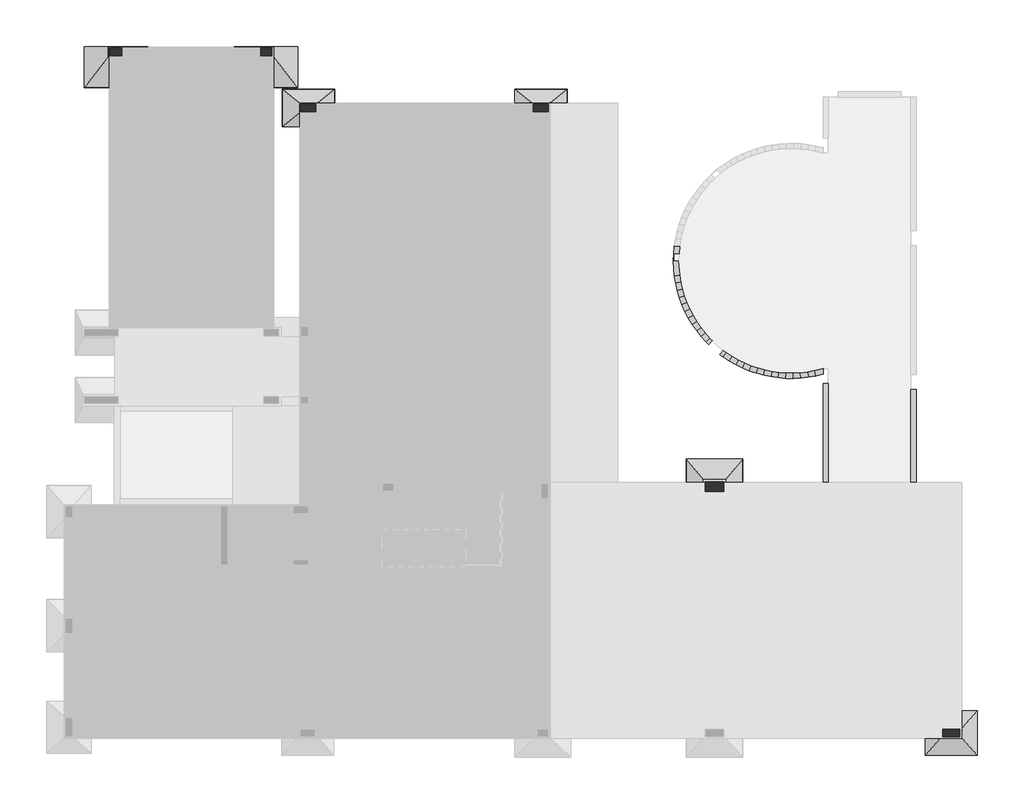
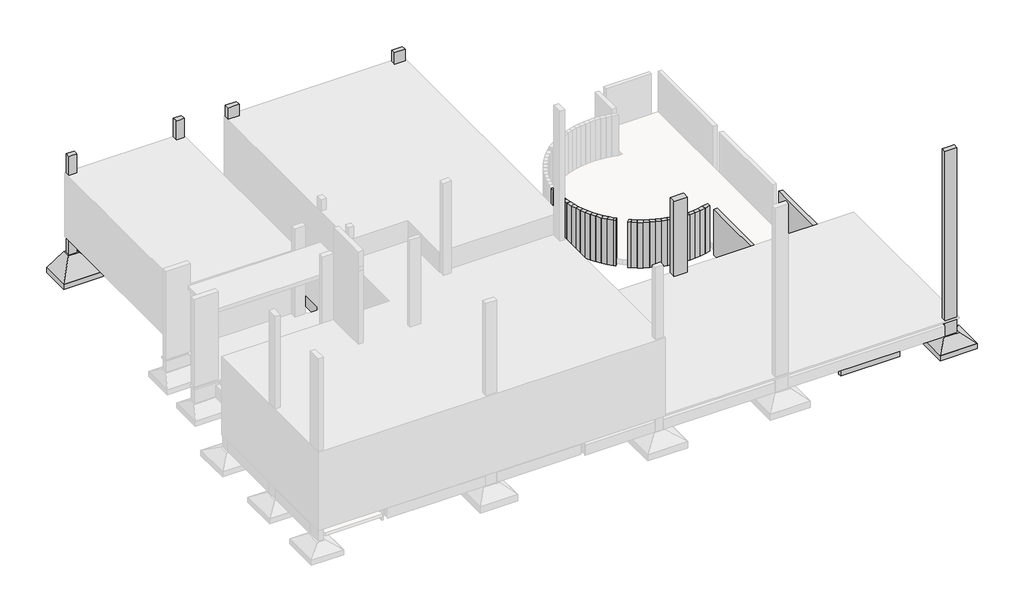
# One storey, part 3 of 4: 35 beams, 7 fasteners, 6 columns.
# Revit data of these elements (continued)
# Type "TQS - Sapata : S2" (continued)
#   H0 = 0.20 m
#   EXCYABS = 0.85 m
#   EXCY = 0.00 m
#   EXCXABS = 0.145 m
#   EXCX = -0.405 m
#   DIMY = 1.70 m
#   DIMX = 1.10 m
#   Material estrutural = Concreto - Concreto concretado no local
#   Width = 0
#   Length = 0
# Type "TQS - Sapata : S24"
#   TY = 0.60 m
#   TX = 0.29 m
#   HS = 0.50 m
#   H0 = 0.20 m
#   EXCYABS = 0.70 m
#   EXCY = 0.00 m
#   EXCXABS = 0.60 m
#   EXCX = 0.00 m
#   DIMY = 1.40 m
#   DIMX = 1.20 m
#   Material estrutural = Concreto - Concreto concretado no local
#   Width = 0
#   Length = 0
# Type "TQS - Sapata : S3"
#   TY = 0.50 m
#   TX = 0.29 m
#   HS = 0.50 m
#   H0 = 0.20 m
#   EXCYABS = 0.70 m
#   EXCY = 0.00 m
#   EXCXABS = 0.50 m
#   EXCX = 0.00 m
#   DIMY = 1.40 m
#   DIMX = 1.00 m
#   Material estrutural = Concreto - Concreto concretado no local
#   Width = 0
#   Length = 0
# Type "TQS - Sapata : S4"
#   TY = 0.50 m
#   TX = 0.29 m
#   HS = 0.50 m
#   H0 = 0.20 m
#   EXCYABS = 0.70 m
#   EXCY = 0.00 m
#   EXCXABS = 0.50 m
#   EXCX = 0.00 m
#   DIMY = 1.40 m
#   DIMX = 1.00 m
#   Material estrutural = Concreto - Concreto concretado no local
#   Width = 0
#   Length = 0
# Element 1 (IfcBeam, "TQS - Viga retangular : 14.0 x 180.0")
#   Uso = "ESTRUTURA"
#   Titulo = "VP2"
#   Chave = "-984"
#   Tipo Elemento = "Viga"
#   SHA1 = "67BB47F7F07D141E1E461B1B62FFCED57BE49A5E"
#   Revisão = ""
#   Tipo de carga = ""
#   Divisor de flexao = ""
#   Secao = ""
#   Configuracao = ""
#   Angulo (graus) = ""
#   Detalhamento = ""
#   Casos de vento manual = ""
#   Tipo = ""
#   Alcas = ""
#   Furos = ""
#   Pino = ""
#   Distribuicao = ""
#   Solidarizado = ""
#   Solidarizar na montagem = ""
#   Unir com o próximo = ""
#   Grupo pre moldado = ""
#   Verificado = ""
#   Concreto C = ""
#   Taxa de armadura (kgf/m³) = 0
#   Carga (tf/m²) = 0
#   Carga (tf/m) = 0
#   Carga (tf) = 0
#   Altura = 1.80 m
#   Rebaixo = 0.15 m
#   Largura = 0.14 m
#   Distancia a face = 0.00 m
#   Distancia ao eixo = 0.00 m
#   Altura gerber esquerda = 0.00 m
#   Largura gerber esquerda = 0.00 m
#   Altura gerber direita = 0.00 m
#   Largura gerber direita = 0.00 m
#   Resultado de Ensaios fck (MPa) = 0
#   Unique TQS ID = -984
#   Principal = yes
#   Structural Material = none
#   Phase Created = CC_AP/ESTR
# Element 2 (IfcBeam, "TQS - Viga retangular : 14.0 x 180.0")
#   Uso = "ESTRUTURA"
#   Titulo = "VP3"
#   Chave = "-985"
#   Tipo Elemento = "Viga"
#   SHA1 = "1D3F2A738C11C779DD3B877E14C8E10A324E012C"
#   Revisão = ""
#   Tipo de carga = ""
#   Divisor de flexao = ""
#   Secao = ""
#   Configuracao = ""
#   Angulo (graus) = ""
#   Detalhamento = ""
#   Casos de vento manual = ""
#   Tipo = ""
#   Alcas = ""
#   Furos = ""
#   Pino = ""
#   Distribuicao = ""
#   Solidarizado = ""
#   Solidarizar na montagem = ""
#   Unir com o próximo = ""
#   Grupo pre moldado = ""
#   Verificado = ""
#   Concreto C = ""
#   Taxa de armadura (kgf/m³) = 0
#   Carga (tf/m²) = 0
#   Carga (tf/m) = 0
#   Carga (tf) = 0
#   Altura = 1.80 m
#   Rebaixo = 0.15 m
#   Largura = 0.14 m
#   Distancia a face = 0.00 m
#   Distancia ao eixo = 0.00 m
#   Altura gerber esquerda = 0.00 m
#   Largura gerber esquerda = 0.00 m
#   Altura gerber direita = 0.00 m
#   Largura gerber direita = 0.00 m
#   Resultado de Ensaios fck (MPa) = 0
#   Unique TQS ID = -985
#   Principal = yes
#   Structural Material = none
#   Phase Created = CC_AP/ESTR
# Element 3 (IfcBeam, "TQS - Viga retangular : 14.0 x 180.0")
#   Uso = "ESTRUTURA"
#   Titulo = "VP4"
#   Chave = "-987"
#   Tipo Elemento = "Viga"
#   SHA1 = "18E803970E3FF61AE3A7C4B8095E8E40226C0AA9"
#   Revisão = ""
#   Tipo de carga = ""
#   Divisor de flexao = ""
#   Secao = ""
#   Configuracao = ""
#   Angulo (graus) = ""
#   Detalhamento = ""
#   Casos de vento manual = ""
#   Tipo = ""
#   Alcas = ""
#   Furos = ""
#   Pino = ""
#   Distribuicao = ""
#   Solidarizado = ""
#   Solidarizar na montagem = ""
#   Unir com o próximo = ""
#   Grupo pre moldado = ""
#   Verificado = ""
#   Concreto C = ""
#   Taxa de armadura (kgf/m³) = 0
#   Carga (tf/m²) = 0
#   Carga (tf/m) = 0
#   Carga (tf) = 0
#   Altura = 1.80 m
#   Rebaixo = 0.15 m
#   Largura = 0.14 m
#   Distancia a face = 0.00 m
#   Distancia ao eixo = 0.00 m
#   Altura gerber esquerda = 0.00 m
#   Largura gerber esquerda = 0.00 m
#   Altura gerber direita = 0.00 m
#   Largura gerber direita = 0.00 m
#   Resultado de Ensaios fck (MPa) = 0
#   Unique TQS ID = -987
#   Principal = yes
#   Structural Material = none
#   Phase Created = CC_AP/ESTR
# Element 4 (IfcBeam, "TQS - Viga retangular : 14.0 x 180.0")
#   Uso = "ESTRUTURA"
#   Titulo = "VP4"
#   Chave = "-988"
#   Tipo Elemento = "Viga"
#   SHA1 = "B71FF30D7224BC3A2F9C0912C04A339394FFFF18"
#   Revisão = ""
#   Tipo de carga = ""
#   Divisor de flexao = ""
#   Secao = ""
#   Configuracao = ""
#   Angulo (graus) = ""
#   Detalhamento = ""
#   Casos de vento manual = ""
#   Tipo = ""
#   Alcas = ""
#   Furos = ""
#   Pino = ""
#   Distribuicao = ""
#   Solidarizado = ""
#   Solidarizar na montagem = ""
#   Unir com o próximo = ""
#   Grupo pre moldado = ""
#   Verificado = ""
#   Concreto C = ""
#   Taxa de armadura (kgf/m³) = 0
#   Carga (tf/m²) = 0
#   Carga (tf/m) = 0
#   Carga (tf) = 0
#   Altura = 1.80 m
#   Rebaixo = 0.15 m
#   Largura = 0.14 m
#   Distancia a face = 0.00 m
#   Distancia ao eixo = 0.00 m
#   Altura gerber esquerda = 0.00 m
#   Largura gerber esquerda = 0.00 m
#   Altura gerber direita = 0.00 m
#   Largura gerber direita = 0.00 m
#   Resultado de Ensaios fck (MPa) = 0
#   Unique TQS ID = -988
#   Principal = yes
#   Structural Material = none
#   Phase Created = CC_AP/ESTR
# Element 5 (IfcBeam, "TQS - Viga retangular : 14.0 x 180.0")
#   Uso = "ESTRUTURA"
#   Titulo = "VP4"
#   Chave = "-989"
#   Tipo Elemento = "Viga"
#   SHA1 = "E9E1B2FEFAB6FC9E808C50FA3A91823AD53CDAD9"
#   Revisão = ""
#   Tipo de carga = ""
#   Divisor de flexao = ""
#   Secao = ""
#   Configuracao = ""
#   Angulo (graus) = ""
#   Detalhamento = ""
#   Casos de vento manual = ""
#   Tipo = ""
#   Alcas = ""
#   Furos = ""
#   Pino = ""
#   Distribuicao = ""
#   Solidarizado = ""
#   Solidarizar na montagem = ""
#   Unir com o próximo = ""
#   Grupo pre moldado = ""
#   Verificado = ""
#   Concreto C = ""
#   Taxa de armadura (kgf/m³) = 0
#   Carga (tf/m²) = 0
#   Carga (tf/m) = 0
#   Carga (tf) = 0
#   Altura = 1.80 m
#   Rebaixo = 0.15 m
#   Largura = 0.14 m
#   Distancia a face = 0.00 m
#   Distancia ao eixo = 0.00 m
#   Altura gerber esquerda = 0.00 m
#   Largura gerber esquerda = 0.00 m
#   Altura gerber direita = 0.00 m
#   Largura gerber direita = 0.00 m
#   Resultado de Ensaios fck (MPa) = 0
#   Unique TQS ID = -989
#   Principal = yes
#   Structural Material = none
#   Phase Created = CC_AP/ESTR
# Element 6 (IfcBeam, "TQS - Viga retangular : 14.0 x 180.0")
#   Uso = "ESTRUTURA"
#   Titulo = "VP4"
#   Chave = "-990"
#   Tipo Elemento = "Viga"
#   SHA1 = "A4F79934EF83F3B7E9A1E2CD35D009C4681F812D"
#   Revisão = ""
#   Tipo de carga = ""
#   Divisor de flexao = ""
#   Secao = ""
#   Configuracao = ""
#   Angulo (graus) = ""
#   Detalhamento = ""
#   Casos de vento manual = ""
#   Tipo = ""
#   Alcas = ""
#   Furos = ""
#   Pino = ""
#   Distribuicao = ""
#   Solidarizado = ""
#   Solidarizar na montagem = ""
#   Unir com o próximo = ""
#   Grupo pre moldado = ""
#   Verificado = ""
#   Concreto C = ""
#   Taxa de armadura (kgf/m³) = 0
#   Carga (tf/m²) = 0
#   Carga (tf/m) = 0
#   Carga (tf) = 0
#   Altura = 1.80 m
#   Rebaixo = 0.15 m
#   Largura = 0.14 m
#   Distancia a face = 0.00 m
#   Distancia ao eixo = 0.00 m
#   Altura gerber esquerda = 0.00 m
#   Largura gerber esquerda = 0.00 m
#   Altura gerber direita = 0.00 m
#   Largura gerber direita = 0.00 m
#   Resultado de Ensaios fck (MPa) = 0
#   Unique TQS ID = -990
#   Principal = yes
#   Structural Material = none
#   Phase Created = CC_AP/ESTR
# Element 7 (IfcBeam, "TQS - Viga retangular : 14.0 x 180.0")
#   Uso = "ESTRUTURA"
#   Titulo = "VP4"
#   Chave = "-991"
#   Tipo Elemento = "Viga"
#   SHA1 = "59C2882C15F8D77C9BC823B17A9B229971BFE292"
#   Revisão = ""
#   Tipo de carga = ""
#   Divisor de flexao = ""
#   Secao = ""
#   Configuracao = ""
#   Angulo (graus) = ""
#   Detalhamento = ""
#   Casos de vento manual = ""
#   Tipo = ""
#   Alcas = ""
#   Furos = ""
#   Pino = ""
#   Distribuicao = ""
#   Solidarizado = ""
#   Solidarizar na montagem = ""
#   Unir com o próximo = ""
#   Grupo pre moldado = ""
#   Verificado = ""
#   Concreto C = ""
#   Taxa de armadura (kgf/m³) = 0
#   Carga (tf/m²) = 0
#   Carga (tf/m) = 0
#   Carga (tf) = 0
#   Altura = 1.80 m
#   Rebaixo = 0.15 m
#   Largura = 0.14 m
#   Distancia a face = 0.00 m
#   Distancia ao eixo = 0.00 m
#   Altura gerber esquerda = 0.00 m
#   Largura gerber esquerda = 0.00 m
#   Altura gerber direita = 0.00 m
#   Largura gerber direita = 0.00 m
#   Resultado de Ensaios fck (MPa) = 0
#   Unique TQS ID = -991
#   Principal = yes
#   Structural Material = none
#   Phase Created = CC_AP/ESTR
# Element 8 (IfcBeam, "TQS - Viga retangular : 14.0 x 180.0")
#   Uso = "ESTRUTURA"
#   Titulo = "VP4"
#   Chave = "-992"
#   Tipo Elemento = "Viga"
#   SHA1 = "6D985E6B9F5FA1FD140F505980BE925AA5C487F2"
#   Revisão = ""
#   Tipo de carga = ""
#   Divisor de flexao = ""
#   Secao = ""
#   Configuracao = ""
#   Angulo (graus) = ""
#   Detalhamento = ""
#   Casos de vento manual = ""
#   Tipo = ""
#   Alcas = ""
#   Furos = ""
#   Pino = ""
#   Distribuicao = ""
#   Solidarizado = ""
#   Solidarizar na montagem = ""
#   Unir com o próximo = ""
#   Grupo pre moldado = ""
#   Verificado = ""
#   Concreto C = ""
#   Taxa de armadura (kgf/m³) = 0
#   Carga (tf/m²) = 0
#   Carga (tf/m) = 0
#   Carga (tf) = 0
#   Altura = 1.80 m
#   Rebaixo = 0.15 m
#   Largura = 0.14 m
#   Distancia a face = 0.00 m
#   Distancia ao eixo = 0.00 m
#   Altura gerber esquerda = 0.00 m
#   Largura gerber esquerda = 0.00 m
#   Altura gerber direita = 0.00 m
#   Largura gerber direita = 0.00 m
#   Resultado de Ensaios fck (MPa) = 0
#   Unique TQS ID = -992
#   Principal = yes
#   Structural Material = none
#   Phase Created = CC_AP/ESTR
# Element 9 (IfcBeam, "TQS - Viga retangular : 14.0 x 180.0")
#   Uso = "ESTRUTURA"
#   Titulo = "VP4"
#   Chave = "-993"
#   Tipo Elemento = "Viga"
#   SHA1 = "5D4E92287FB362FDFCD64B2B7E6C35302CB92A79"
#   Revisão = ""
#   Tipo de carga = ""
#   Divisor de flexao = ""
#   Secao = ""
#   Configuracao = ""
#   Angulo (graus) = ""
#   Detalhamento = ""
#   Casos de vento manual = ""
#   Tipo = ""
#   Alcas = ""
#   Furos = ""
#   Pino = ""
#   Distribuicao = ""
#   Solidarizado = ""
#   Solidarizar na montagem = ""
#   Unir com o próximo = ""
#   Grupo pre moldado = ""
#   Verificado = ""
#   Concreto C = ""
#   Taxa de armadura (kgf/m³) = 0
#   Carga (tf/m²) = 0
#   Carga (tf/m) = 0
#   Carga (tf) = 0
#   Altura = 1.80 m
#   Rebaixo = 0.15 m
#   Largura = 0.14 m
#   Distancia a face = 0.00 m
#   Distancia ao eixo = 0.00 m
#   Altura gerber esquerda = 0.00 m
#   Largura gerber esquerda = 0.00 m
#   Altura gerber direita = 0.00 m
#   Largura gerber direita = 0.00 m
#   Resultado de Ensaios fck (MPa) = 0
#   Unique TQS ID = -993
#   Principal = yes
#   Structural Material = none
#   Phase Created = CC_AP/ESTR
# Element 10 (IfcBeam, "TQS - Viga retangular : 14.0 x 180.0")
#   Uso = "ESTRUTURA"
#   Titulo = "VP4"
#   Chave = "-994"
#   Tipo Elemento = "Viga"
#   SHA1 = "B241F61C6536B176DF9E3A8727FE075D16BE7057"
#   Revisão = ""
#   Tipo de carga = ""
#   Divisor de flexao = ""
#   Secao = ""
#   Configuracao = ""
#   Angulo (graus) = ""
#   Detalhamento = ""
#   Casos de vento manual = ""
#   Tipo = ""
#   Alcas = ""
#   Furos = ""
#   Pino = ""
#   Distribuicao = ""
#   Solidarizado = ""
#   Solidarizar na montagem = ""
#   Unir com o próximo = ""
#   Grupo pre moldado = ""
#   Verificado = ""
#   Concreto C = ""
#   Taxa de armadura (kgf/m³) = 0
#   Carga (tf/m²) = 0
#   Carga (tf/m) = 0
#   Carga (tf) = 0
#   Altura = 1.80 m
#   Rebaixo = 0.15 m
#   Largura = 0.14 m
#   Distancia a face = 0.00 m
#   Distancia ao eixo = 0.00 m
#   Altura gerber esquerda = 0.00 m
#   Largura gerber esquerda = 0.00 m
#   Altura gerber direita = 0.00 m
#   Largura gerber direita = 0.00 m
#   Resultado de Ensaios fck (MPa) = 0
#   Unique TQS ID = -994
#   Principal = yes
#   Structural Material = none
#   Phase Created = CC_AP/ESTR
# Element 11 (IfcBeam, "TQS - Viga retangular : 14.0 x 180.0")
#   Uso = "ESTRUTURA"
#   Titulo = "VP4"
#   Chave = "-995"
#   Tipo Elemento = "Viga"
#   SHA1 = "79F2E8F443EC2E8CC5B8F506A3E5025E7F953CE7"
#   Revisão = ""
#   Tipo de carga = ""
#   Divisor de flexao = ""
#   Secao = ""
#   Configuracao = ""
#   Angulo (graus) = ""
#   Detalhamento = ""
#   Casos de vento manual = ""
#   Tipo = ""
#   Alcas = ""
#   Furos = ""
#   Pino = ""
#   Distribuicao = ""
#   Solidarizado = ""
#   Solidarizar na montagem = ""
#   Unir com o próximo = ""
#   Grupo pre moldado = ""
#   Verificado = ""
#   Concreto C = ""
#   Taxa de armadura (kgf/m³) = 0
#   Carga (tf/m²) = 0
#   Carga (tf/m) = 0
#   Carga (tf) = 0
#   Altura = 1.80 m
#   Rebaixo = 0.15 m
#   Largura = 0.14 m
#   Distancia a face = 0.00 m
#   Distancia ao eixo = 0.00 m
#   Altura gerber esquerda = 0.00 m
#   Largura gerber esquerda = 0.00 m
#   Altura gerber direita = 0.00 m
#   Largura gerber direita = 0.00 m
#   Resultado de Ensaios fck (MPa) = 0
#   Unique TQS ID = -995
#   Principal = yes
#   Structural Material = none
#   Phase Created = CC_AP/ESTR
# Element 12 (IfcBeam, "TQS - Viga retangular : 14.0 x 180.0")
#   Uso = "ESTRUTURA"
#   Titulo = "VP4"
#   Chave = "-996"
#   Tipo Elemento = "Viga"
#   SHA1 = "EC69CF733B6B75DD72A616518C986B1D4EC6373A"
#   Revisão = ""
#   Tipo de carga = ""
#   Divisor de flexao = ""
#   Secao = ""
#   Configuracao = ""
#   Angulo (graus) = ""
#   Detalhamento = ""
#   Casos de vento manual = ""
#   Tipo = ""
#   Alcas = ""
#   Furos = ""
#   Pino = ""
#   Distribuicao = ""
#   Solidarizado = ""
#   Solidarizar na montagem = ""
#   Unir com o próximo = ""
#   Grupo pre moldado = ""
#   Verificado = ""
#   Concreto C = ""
#   Taxa de armadura (kgf/m³) = 0
#   Carga (tf/m²) = 0
#   Carga (tf/m) = 0
#   Carga (tf) = 0
#   Altura = 1.80 m
#   Rebaixo = 0.15 m
#   Largura = 0.14 m
#   Distancia a face = 0.00 m
#   Distancia ao eixo = 0.00 m
#   Altura gerber esquerda = 0.00 m
#   Largura gerber esquerda = 0.00 m
#   Altura gerber direita = 0.00 m
#   Largura gerber direita = 0.00 m
#   Resultado de Ensaios fck (MPa) = 0
#   Unique TQS ID = -996
#   Principal = yes
#   Structural Material = none
#   Phase Created = CC_AP/ESTR
# Element 13 (IfcBeam, "TQS - Viga retangular : 14.0 x 180.0")
#   Uso = "ESTRUTURA"
#   Titulo = "VP4"
#   Chave = "-997"
#   Tipo Elemento = "Viga"
#   SHA1 = "A94BB0AB94C95055560F49AF3BCE408F9E38B8C0"
#   Revisão = ""
#   Tipo de carga = ""
#   Divisor de flexao = ""
#   Secao = ""
#   Configuracao = ""
#   Angulo (graus) = ""
#   Detalhamento = ""
#   Casos de vento manual = ""
#   Tipo = ""
#   Alcas = ""
#   Furos = ""
#   Pino = ""
#   Distribuicao = ""
#   Solidarizado = ""
#   Solidarizar na montagem = ""
#   Unir com o próximo = ""
#   Grupo pre moldado = ""
#   Verificado = ""
#   Concreto C = ""
#   Taxa de armadura (kgf/m³) = 0
#   Carga (tf/m²) = 0
#   Carga (tf/m) = 0
#   Carga (tf) = 0
#   Altura = 1.80 m
#   Rebaixo = 0.15 m
#   Largura = 0.14 m
#   Distancia a face = 0.00 m
#   Distancia ao eixo = 0.00 m
#   Altura gerber esquerda = 0.00 m
#   Largura gerber esquerda = 0.00 m
#   Altura gerber direita = 0.00 m
#   Largura gerber direita = 0.00 m
#   Resultado de Ensaios fck (MPa) = 0
#   Unique TQS ID = -997
#   Principal = yes
#   Structural Material = none
#   Phase Created = CC_AP/ESTR
# Element 14 (IfcBeam, "TQS - Viga retangular : 14.0 x 180.0")
#   Uso = "ESTRUTURA"
#   Titulo = "VP4"
#   Chave = "-998"
#   Tipo Elemento = "Viga"
#   SHA1 = "6378FB8D39603434150BF0AD569D703CFB80FE5F"
#   Revisão = ""
#   Tipo de carga = ""
#   Divisor de flexao = ""
#   Secao = ""
#   Configuracao = ""
#   Angulo (graus) = ""
#   Detalhamento = ""
#   Casos de vento manual = ""
#   Tipo = ""
#   Alcas = ""
#   Furos = ""
#   Pino = ""
#   Distribuicao = ""
#   Solidarizado = ""
#   Solidarizar na montagem = ""
#   Unir com o próximo = ""
#   Grupo pre moldado = ""
#   Verificado = ""
#   Concreto C = ""
#   Taxa de armadura (kgf/m³) = 0
#   Carga (tf/m²) = 0
#   Carga (tf/m) = 0
#   Carga (tf) = 0
#   Altura = 1.80 m
#   Rebaixo = 0.15 m
#   Largura = 0.14 m
#   Distancia a face = 0.00 m
#   Distancia ao eixo = 0.00 m
#   Altura gerber esquerda = 0.00 m
#   Largura gerber esquerda = 0.00 m
#   Altura gerber direita = 0.00 m
#   Largura gerber direita = 0.00 m
#   Resultado de Ensaios fck (MPa) = 0
#   Unique TQS ID = -998
#   Principal = yes
#   Structural Material = none
#   Phase Created = CC_AP/ESTR
# Element 15 (IfcBeam, "TQS - Viga retangular : 14.0 x 180.0")
#   Uso = "ESTRUTURA"
#   Titulo = "VP4"
#   Chave = "-999"
#   Tipo Elemento = "Viga"
#   SHA1 = "2B4C78D211D826E735DAAC0C825AB5B97130EBCE"
#   Revisão = ""
#   Tipo de carga = ""
#   Divisor de flexao = ""
#   Secao = ""
#   Configuracao = ""
#   Angulo (graus) = ""
#   Detalhamento = ""
#   Casos de vento manual = ""
#   Tipo = ""
#   Alcas = ""
#   Furos = ""
#   Pino = ""
#   Distribuicao = ""
#   Solidarizado = ""
#   Solidarizar na montagem = ""
#   Unir com o próximo = ""
#   Grupo pre moldado = ""
#   Verificado = ""
#   Concreto C = ""
#   Taxa de armadura (kgf/m³) = 0
#   Carga (tf/m²) = 0
#   Carga (tf/m) = 0
#   Carga (tf) = 0
#   Altura = 1.80 m
#   Rebaixo = 0.15 m
#   Largura = 0.14 m
#   Distancia a face = 0.00 m
#   Distancia ao eixo = 0.00 m
#   Altura gerber esquerda = 0.00 m
#   Largura gerber esquerda = 0.00 m
#   Altura gerber direita = 0.00 m
#   Largura gerber direita = 0.00 m
#   Resultado de Ensaios fck (MPa) = 0
#   Unique TQS ID = -999
#   Principal = yes
#   Structural Material = none
#   Phase Created = CC_AP/ESTR
# Element 16 (IfcBeam, "TQS - Viga retangular : 14.0 x 180.0")
#   Uso = "ESTRUTURA"
#   Titulo = "VP4"
#   Chave = "-1000"
#   Tipo Elemento = "Viga"
#   SHA1 = "DD50D292EAFD20D7EF85643CCD075ACF91033CA0"
#   Revisão = ""
#   Tipo de carga = ""
#   Divisor de flexao = ""
#   Secao = ""
#   Configuracao = ""
#   Angulo (graus) = ""
#   Detalhamento = ""
#   Casos de vento manual = ""
#   Tipo = ""
#   Alcas = ""
#   Furos = ""
#   Pino = ""
#   Distribuicao = ""
#   Solidarizado = ""
#   Solidarizar na montagem = ""
#   Unir com o próximo = ""
#   Grupo pre moldado = ""
#   Verificado = ""
#   Concreto C = ""
#   Taxa de armadura (kgf/m³) = 0
#   Carga (tf/m²) = 0
#   Carga (tf/m) = 0
#   Carga (tf) = 0
#   Altura = 1.80 m
#   Rebaixo = 0.15 m
#   Largura = 0.14 m
#   Distancia a face = 0.00 m
#   Distancia ao eixo = 0.00 m
#   Altura gerber esquerda = 0.00 m
#   Largura gerber esquerda = 0.00 m
#   Altura gerber direita = 0.00 m
#   Largura gerber direita = 0.00 m
#   Resultado de Ensaios fck (MPa) = 0
#   Unique TQS ID = -1000
#   Principal = yes
#   Structural Material = none
#   Phase Created = CC_AP/ESTR
# Element 17 (IfcBeam, "TQS - Viga retangular : 14.0 x 180.0")
#   Uso = "ESTRUTURA"
#   Titulo = "VP4"
#   Chave = "-1001"
#   Tipo Elemento = "Viga"
#   SHA1 = "17AE169FA700E73A155B49B14AA872A50BD18F4B"
#   Revisão = ""
#   Tipo de carga = ""
#   Divisor de flexao = ""
#   Secao = ""
#   Configuracao = ""
#   Angulo (graus) = ""
#   Detalhamento = ""
#   Casos de vento manual = ""
#   Tipo = ""
#   Alcas = ""
#   Furos = ""
#   Pino = ""
#   Distribuicao = ""
#   Solidarizado = ""
#   Solidarizar na montagem = ""
#   Unir com o próximo = ""
#   Grupo pre moldado = ""
#   Verificado = ""
#   Concreto C = ""
#   Taxa de armadura (kgf/m³) = 0
#   Carga (tf/m²) = 0
#   Carga (tf/m) = 0
#   Carga (tf) = 0
#   Altura = 1.80 m
#   Rebaixo = 0.15 m
#   Largura = 0.14 m
#   Distancia a face = 0.00 m
#   Distancia ao eixo = 0.00 m
#   Altura gerber esquerda = 0.00 m
#   Largura gerber esquerda = 0.00 m
#   Altura gerber direita = 0.00 m
#   Largura gerber direita = 0.00 m
#   Resultado de Ensaios fck (MPa) = 0
#   Unique TQS ID = -1001
#   Principal = yes
#   Structural Material = none
#   Phase Created = CC_AP/ESTR
# Element 18 (IfcBeam, "TQS - Viga retangular : 14.0 x 180.0")
#   Uso = "ESTRUTURA"
#   Titulo = "VP5"
#   Chave = "-1002"
#   Tipo Elemento = "Viga"
#   SHA1 = "4C02C5B53EDBB34F44F4EAF2E9EE20AD89CC6C79"
#   Revisão = ""
#   Tipo de carga = ""
#   Divisor de flexao = ""
#   Secao = ""
#   Configuracao = ""
#   Angulo (graus) = ""
#   Detalhamento = ""
#   Casos de vento manual = ""
#   Tipo = ""
#   Alcas = ""
#   Furos = ""
#   Pino = ""
#   Distribuicao = ""
#   Solidarizado = ""
#   Solidarizar na montagem = ""
#   Unir com o próximo = ""
#   Grupo pre moldado = ""
#   Verificado = ""
#   Concreto C = ""
#   Taxa de armadura (kgf/m³) = 0
#   Carga (tf/m²) = 0
#   Carga (tf/m) = 0
#   Carga (tf) = 0
#   Altura = 1.80 m
#   Rebaixo = 0.15 m
#   Largura = 0.14 m
#   Distancia a face = 0.00 m
#   Distancia ao eixo = 0.00 m
#   Altura gerber esquerda = 0.00 m
#   Largura gerber esquerda = 0.00 m
#   Altura gerber direita = 0.00 m
#   Largura gerber direita = 0.00 m
#   Resultado de Ensaios fck (MPa) = 0
#   Unique TQS ID = -1002
#   Principal = yes
#   Structural Material = none
#   Phase Created = CC_AP/ESTR
# Element 19 (IfcBeam, "TQS - Viga retangular : 14.0 x 180.0")
#   Uso = "ESTRUTURA"
#   Titulo = "VP5"
#   Chave = "-1003"
#   Tipo Elemento = "Viga"
#   SHA1 = "4CC80C174DC5A33A4959CFE9988141447D2CA55C"
#   Revisão = ""
#   Tipo de carga = ""
#   Divisor de flexao = ""
#   Secao = ""
#   Configuracao = ""
#   Angulo (graus) = ""
#   Detalhamento = ""
#   Casos de vento manual = ""
#   Tipo = ""
#   Alcas = ""
#   Furos = ""
#   Pino = ""
#   Distribuicao = ""
#   Solidarizado = ""
#   Solidarizar na montagem = ""
#   Unir com o próximo = ""
#   Grupo pre moldado = ""
#   Verificado = ""
#   Concreto C = ""
#   Taxa de armadura (kgf/m³) = 0
#   Carga (tf/m²) = 0
#   Carga (tf/m) = 0
#   Carga (tf) = 0
#   Altura = 1.80 m
#   Rebaixo = 0.15 m
#   Largura = 0.14 m
#   Distancia a face = 0.00 m
#   Distancia ao eixo = 0.00 m
#   Altura gerber esquerda = 0.00 m
#   Largura gerber esquerda = 0.00 m
#   Altura gerber direita = 0.00 m
#   Largura gerber direita = 0.00 m
#   Resultado de Ensaios fck (MPa) = 0
#   Unique TQS ID = -1003
#   Principal = yes
#   Structural Material = none
#   Phase Created = CC_AP/ESTR
# Element 20 (IfcBeam, "TQS - Viga retangular : 14.0 x 180.0")
#   Uso = "ESTRUTURA"
#   Titulo = "VP5"
#   Chave = "-1004"
#   Tipo Elemento = "Viga"
#   SHA1 = "B47BB11AE5BEE4DA1AC1C982C2FC48DC4A5ED7AF"
#   Revisão = ""
#   Tipo de carga = ""
#   Divisor de flexao = ""
#   Secao = ""
#   Configuracao = ""
#   Angulo (graus) = ""
#   Detalhamento = ""
#   Casos de vento manual = ""
#   Tipo = ""
#   Alcas = ""
#   Furos = ""
#   Pino = ""
#   Distribuicao = ""
#   Solidarizado = ""
#   Solidarizar na montagem = ""
#   Unir com o próximo = ""
#   Grupo pre moldado = ""
#   Verificado = ""
#   Concreto C = ""
#   Taxa de armadura (kgf/m³) = 0
#   Carga (tf/m²) = 0
#   Carga (tf/m) = 0
#   Carga (tf) = 0
#   Altura = 1.80 m
#   Rebaixo = 0.15 m
#   Largura = 0.14 m
#   Distancia a face = 0.00 m
#   Distancia ao eixo = 0.00 m
#   Altura gerber esquerda = 0.00 m
#   Largura gerber esquerda = 0.00 m
#   Altura gerber direita = 0.00 m
#   Largura gerber direita = 0.00 m
#   Resultado de Ensaios fck (MPa) = 0
#   Unique TQS ID = -1004
#   Principal = yes
#   Structural Material = none
#   Phase Created = CC_AP/ESTR
# Element 21 (IfcBeam, "TQS - Viga retangular : 14.0 x 180.0")
#   Uso = "ESTRUTURA"
#   Titulo = "VP5"
#   Chave = "-1005"
#   Tipo Elemento = "Viga"
#   SHA1 = "D99F413EAFADC372BC776638DB624CCF8BA82056"
#   Revisão = ""
#   Tipo de carga = ""
#   Divisor de flexao = ""
#   Secao = ""
#   Configuracao = ""
#   Angulo (graus) = ""
#   Detalhamento = ""
#   Casos de vento manual = ""
#   Tipo = ""
#   Alcas = ""
#   Furos = ""
#   Pino = ""
#   Distribuicao = ""
#   Solidarizado = ""
#   Solidarizar na montagem = ""
#   Unir com o próximo = ""
#   Grupo pre moldado = ""
#   Verificado = ""
#   Concreto C = ""
#   Taxa de armadura (kgf/m³) = 0
#   Carga (tf/m²) = 0
#   Carga (tf/m) = 0
#   Carga (tf) = 0
#   Altura = 1.80 m
#   Rebaixo = 0.15 m
#   Largura = 0.14 m
#   Distancia a face = 0.00 m
#   Distancia ao eixo = 0.00 m
#   Altura gerber esquerda = 0.00 m
#   Largura gerber esquerda = 0.00 m
#   Altura gerber direita = 0.00 m
#   Largura gerber direita = 0.00 m
#   Resultado de Ensaios fck (MPa) = 0
#   Unique TQS ID = -1005
#   Principal = yes
#   Structural Material = none
#   Phase Created = CC_AP/ESTR
# Element 22 (IfcBeam, "TQS - Viga retangular : 14.0 x 180.0")
#   Uso = "ESTRUTURA"
#   Titulo = "VP5"
#   Chave = "-1006"
#   Tipo Elemento = "Viga"
#   SHA1 = "45441B0255AB8A379653287FCCEE7CF9E9C67E02"
#   Revisão = ""
#   Tipo de carga = ""
#   Divisor de flexao = ""
#   Secao = ""
#   Configuracao = ""
#   Angulo (graus) = ""
#   Detalhamento = ""
#   Casos de vento manual = ""
#   Tipo = ""
#   Alcas = ""
#   Furos = ""
#   Pino = ""
#   Distribuicao = ""
#   Solidarizado = ""
#   Solidarizar na montagem = ""
#   Unir com o próximo = ""
#   Grupo pre moldado = ""
#   Verificado = ""
#   Concreto C = ""
#   Taxa de armadura (kgf/m³) = 0
#   Carga (tf/m²) = 0
#   Carga (tf/m) = 0
#   Carga (tf) = 0
#   Altura = 1.80 m
#   Rebaixo = 0.15 m
#   Largura = 0.14 m
#   Distancia a face = 0.00 m
#   Distancia ao eixo = 0.00 m
#   Altura gerber esquerda = 0.00 m
#   Largura gerber esquerda = 0.00 m
#   Altura gerber direita = 0.00 m
#   Largura gerber direita = 0.00 m
#   Resultado de Ensaios fck (MPa) = 0
#   Unique TQS ID = -1006
#   Principal = yes
#   Structural Material = none
#   Phase Created = CC_AP/ESTR
# Element 23 (IfcBeam, "TQS - Viga retangular : 14.0 x 180.0")
#   Uso = "ESTRUTURA"
#   Titulo = "VP5"
#   Chave = "-1007"
#   Tipo Elemento = "Viga"
#   SHA1 = "67D8F0B72EA773B01EE7283A9BF6FD7CCC373B16"
#   Revisão = ""
#   Tipo de carga = ""
#   Divisor de flexao = ""
#   Secao = ""
#   Configuracao = ""
#   Angulo (graus) = ""
#   Detalhamento = ""
#   Casos de vento manual = ""
#   Tipo = ""
#   Alcas = ""
#   Furos = ""
#   Pino = ""
#   Distribuicao = ""
#   Solidarizado = ""
#   Solidarizar na montagem = ""
#   Unir com o próximo = ""
#   Grupo pre moldado = ""
#   Verificado = ""
#   Concreto C = ""
#   Taxa de armadura (kgf/m³) = 0
#   Carga (tf/m²) = 0
#   Carga (tf/m) = 0
#   Carga (tf) = 0
#   Altura = 1.80 m
#   Rebaixo = 0.15 m
#   Largura = 0.14 m
#   Distancia a face = 0.00 m
#   Distancia ao eixo = 0.00 m
#   Altura gerber esquerda = 0.00 m
#   Largura gerber esquerda = 0.00 m
#   Altura gerber direita = 0.00 m
#   Largura gerber direita = 0.00 m
#   Resultado de Ensaios fck (MPa) = 0
#   Unique TQS ID = -1007
#   Principal = yes
#   Structural Material = none
#   Phase Created = CC_AP/ESTR
# Element 24 (IfcBeam, "TQS - Viga retangular : 14.0 x 180.0")
#   Uso = "ESTRUTURA"
#   Titulo = "VP5"
#   Chave = "-1008"
#   Tipo Elemento = "Viga"
#   SHA1 = "97D86C514C265A9FC3405D75886B30F1FDE07F5F"
#   Revisão = ""
#   Tipo de carga = ""
#   Divisor de flexao = ""
#   Secao = ""
#   Configuracao = ""
#   Angulo (graus) = ""
#   Detalhamento = ""
#   Casos de vento manual = ""
#   Tipo = ""
#   Alcas = ""
#   Furos = ""
#   Pino = ""
#   Distribuicao = ""
#   Solidarizado = ""
#   Solidarizar na montagem = ""
#   Unir com o próximo = ""
#   Grupo pre moldado = ""
#   Verificado = ""
#   Concreto C = ""
#   Taxa de armadura (kgf/m³) = 0
#   Carga (tf/m²) = 0
#   Carga (tf/m) = 0
#   Carga (tf) = 0
#   Altura = 1.80 m
#   Rebaixo = 0.15 m
#   Largura = 0.14 m
#   Distancia a face = 0.00 m
#   Distancia ao eixo = 0.00 m
#   Altura gerber esquerda = 0.00 m
#   Largura gerber esquerda = 0.00 m
#   Altura gerber direita = 0.00 m
#   Largura gerber direita = 0.00 m
#   Resultado de Ensaios fck (MPa) = 0
#   Unique TQS ID = -1008
#   Principal = yes
#   Structural Material = none
#   Phase Created = CC_AP/ESTR
# Element 25 (IfcBeam, "TQS - Viga retangular : 14.0 x 180.0")
#   Uso = "ESTRUTURA"
#   Titulo = "VP5"
#   Chave = "-1009"
#   Tipo Elemento = "Viga"
#   SHA1 = "E11E876F0FB2670C71699C66FE517DB49DCFCCF5"
#   Revisão = ""
#   Tipo de carga = ""
#   Divisor de flexao = ""
#   Secao = ""
#   Configuracao = ""
#   Angulo (graus) = ""
#   Detalhamento = ""
#   Casos de vento manual = ""
#   Tipo = ""
#   Alcas = ""
#   Furos = ""
#   Pino = ""
#   Distribuicao = ""
#   Solidarizado = ""
#   Solidarizar na montagem = ""
#   Unir com o próximo = ""
#   Grupo pre moldado = ""
#   Verificado = ""
#   Concreto C = ""
#   Taxa de armadura (kgf/m³) = 0
#   Carga (tf/m²) = 0
#   Carga (tf/m) = 0
#   Carga (tf) = 0
#   Altura = 1.80 m
#   Rebaixo = 0.15 m
#   Largura = 0.14 m
#   Distancia a face = 0.00 m
#   Distancia ao eixo = 0.00 m
#   Altura gerber esquerda = 0.00 m
#   Largura gerber esquerda = 0.00 m
#   Altura gerber direita = 0.00 m
#   Largura gerber direita = 0.00 m
#   Resultado de Ensaios fck (MPa) = 0
#   Unique TQS ID = -1009
#   Principal = yes
#   Structural Material = none
#   Phase Created = CC_AP/ESTR
# Element 26 (IfcBeam, "TQS - Viga retangular : 14.0 x 180.0")
#   Uso = "ESTRUTURA"
#   Titulo = "VP5"
#   Chave = "-1010"
#   Tipo Elemento = "Viga"
#   SHA1 = "B2FE66282E83D533D9B7EA94ACB770D2301BAEA7"
#   Revisão = ""
#   Tipo de carga = ""
#   Divisor de flexao = ""
#   Secao = ""
#   Configuracao = ""
#   Angulo (graus) = ""
#   Detalhamento = ""
#   Casos de vento manual = ""
#   Tipo = ""
#   Alcas = ""
#   Furos = ""
#   Pino = ""
#   Distribuicao = ""
#   Solidarizado = ""
#   Solidarizar na montagem = ""
#   Unir com o próximo = ""
#   Grupo pre moldado = ""
#   Verificado = ""
#   Concreto C = ""
#   Taxa de armadura (kgf/m³) = 0
#   Carga (tf/m²) = 0
#   Carga (tf/m) = 0
#   Carga (tf) = 0
#   Altura = 1.80 m
#   Rebaixo = 0.15 m
#   Largura = 0.14 m
#   Distancia a face = 0.00 m
#   Distancia ao eixo = 0.00 m
#   Altura gerber esquerda = 0.00 m
#   Largura gerber esquerda = 0.00 m
#   Altura gerber direita = 0.00 m
#   Largura gerber direita = 0.00 m
#   Resultado de Ensaios fck (MPa) = 0
#   Unique TQS ID = -1010
#   Principal = yes
#   Structural Material = none
#   Phase Created = CC_AP/ESTR
# Element 27 (IfcBeam, "TQS - Viga retangular : 14.0 x 180.0")
#   Uso = "ESTRUTURA"
#   Titulo = "VP5"
#   Chave = "-1011"
#   Tipo Elemento = "Viga"
#   SHA1 = "B326764AED5F8992A99CC84B56FBCB9058379F2E"
#   Revisão = ""
#   Tipo de carga = ""
#   Divisor de flexao = ""
#   Secao = ""
#   Configuracao = ""
#   Angulo (graus) = ""
#   Detalhamento = ""
#   Casos de vento manual = ""
#   Tipo = ""
#   Alcas = ""
#   Furos = ""
#   Pino = ""
#   Distribuicao = ""
#   Solidarizado = ""
#   Solidarizar na montagem = ""
#   Unir com o próximo = ""
#   Grupo pre moldado = ""
#   Verificado = ""
#   Concreto C = ""
#   Taxa de armadura (kgf/m³) = 0
#   Carga (tf/m²) = 0
#   Carga (tf/m) = 0
#   Carga (tf) = 0
#   Altura = 1.80 m
#   Rebaixo = 0.15 m
#   Largura = 0.14 m
#   Distancia a face = 0.00 m
#   Distancia ao eixo = 0.00 m
#   Altura gerber esquerda = 0.00 m
#   Largura gerber esquerda = 0.00 m
#   Altura gerber direita = 0.00 m
#   Largura gerber direita = 0.00 m
#   Resultado de Ensaios fck (MPa) = 0
#   Unique TQS ID = -1011
#   Principal = yes
#   Structural Material = none
#   Phase Created = CC_AP/ESTR
# Element 28 (IfcBeam, "TQS - Viga retangular : 14.0 x 180.0")
#   Uso = "ESTRUTURA"
#   Titulo = "VP5"
#   Chave = "-1012"
#   Tipo Elemento = "Viga"
#   SHA1 = "ADF8088E05543C33AE80BF92F8ECBD3B445E80A1"
#   Revisão = ""
#   Tipo de carga = ""
#   Divisor de flexao = ""
#   Secao = ""
#   Configuracao = ""
#   Angulo (graus) = ""
#   Detalhamento = ""
#   Casos de vento manual = ""
#   Tipo = ""
#   Alcas = ""
#   Furos = ""
#   Pino = ""
#   Distribuicao = ""
#   Solidarizado = ""
#   Solidarizar na montagem = ""
#   Unir com o próximo = ""
#   Grupo pre moldado = ""
#   Verificado = ""
#   Concreto C = ""
#   Taxa de armadura (kgf/m³) = 0
#   Carga (tf/m²) = 0
#   Carga (tf/m) = 0
#   Carga (tf) = 0
#   Altura = 1.80 m
#   Rebaixo = 0.15 m
#   Largura = 0.14 m
#   Distancia a face = 0.00 m
#   Distancia ao eixo = 0.00 m
#   Altura gerber esquerda = 0.00 m
#   Largura gerber esquerda = 0.00 m
#   Altura gerber direita = 0.00 m
#   Largura gerber direita = 0.00 m
#   Resultado de Ensaios fck (MPa) = 0
#   Unique TQS ID = -1012
#   Principal = yes
#   Structural Material = none
#   Phase Created = CC_AP/ESTR
# Element 29 (IfcBeam, "TQS - Viga retangular : 14.0 x 180.0")
#   Uso = "ESTRUTURA"
#   Titulo = "VP5"
#   Chave = "-1013"
#   Tipo Elemento = "Viga"
#   SHA1 = "F629BC16B5B7CEFABB33876C532E6A3B47A757C7"
#   Revisão = ""
#   Tipo de carga = ""
#   Divisor de flexao = ""
#   Secao = ""
#   Configuracao = ""
#   Angulo (graus) = ""
#   Detalhamento = ""
#   Casos de vento manual = ""
#   Tipo = ""
#   Alcas = ""
#   Furos = ""
#   Pino = ""
#   Distribuicao = ""
#   Solidarizado = ""
#   Solidarizar na montagem = ""
#   Unir com o próximo = ""
#   Grupo pre moldado = ""
#   Verificado = ""
#   Concreto C = ""
#   Taxa de armadura (kgf/m³) = 0
#   Carga (tf/m²) = 0
#   Carga (tf/m) = 0
#   Carga (tf) = 0
#   Altura = 1.80 m
#   Rebaixo = 0.15 m
#   Largura = 0.14 m
#   Distancia a face = 0.00 m
#   Distancia ao eixo = 0.00 m
#   Altura gerber esquerda = 0.00 m
#   Largura gerber esquerda = 0.00 m
#   Altura gerber direita = 0.00 m
#   Largura gerber direita = 0.00 m
#   Resultado de Ensaios fck (MPa) = 0
#   Unique TQS ID = -1013
#   Principal = yes
#   Structural Material = none
#   Phase Created = CC_AP/ESTR
# Element 30 (IfcBeam, "TQS - Viga retangular : 14.0 x 180.0")
#   Uso = "ESTRUTURA"
#   Titulo = "VP6"
#   Chave = "-1014"
#   Tipo Elemento = "Viga"
#   SHA1 = "803FE0467B8784052CD3520716E944CE5BCDE54C"
#   Revisão = ""
#   Tipo de carga = ""
#   Divisor de flexao = ""
#   Secao = ""
#   Configuracao = ""
#   Angulo (graus) = ""
#   Detalhamento = ""
#   Casos de vento manual = ""
#   Tipo = ""
#   Alcas = ""
#   Furos = ""
#   Pino = ""
#   Distribuicao = ""
#   Solidarizado = ""
#   Solidarizar na montagem = ""
#   Unir com o próximo = ""
#   Grupo pre moldado = ""
#   Verificado = ""
#   Concreto C = ""
#   Taxa de armadura (kgf/m³) = 0
#   Carga (tf/m²) = 0
#   Carga (tf/m) = 0
#   Carga (tf) = 0
#   Altura = 1.80 m
#   Rebaixo = 0.15 m
#   Largura = 0.14 m
#   Distancia a face = 0.00 m
#   Distancia ao eixo = 0.00 m
#   Altura gerber esquerda = 0.00 m
#   Largura gerber esquerda = 0.00 m
#   Altura gerber direita = 0.00 m
#   Largura gerber direita = 0.00 m
#   Resultado de Ensaios fck (MPa) = 0
#   Unique TQS ID = -1014
#   Principal = yes
#   Structural Material = none
#   Phase Created = CC_AP/ESTR
# Element 31 (IfcBeam, "TQS - Viga retangular : 14.0 x 180.0")
#   Uso = "ESTRUTURA"
#   Titulo = "VP9"
#   Chave = "-1042"
#   Tipo Elemento = "Viga"
#   SHA1 = "A33BDDD61DCA14C8FF84777102E10ABF9273446C"
#   Revisão = ""
#   Tipo de carga = ""
#   Divisor de flexao = ""
#   Secao = ""
#   Configuracao = ""
#   Angulo (graus) = ""
#   Detalhamento = ""
#   Casos de vento manual = ""
#   Tipo = ""
#   Alcas = ""
#   Furos = ""
#   Pino = ""
#   Distribuicao = ""
#   Solidarizado = ""
#   Solidarizar na montagem = ""
#   Unir com o próximo = ""
#   Grupo pre moldado = ""
#   Verificado = ""
#   Concreto C = ""
#   Taxa de armadura (kgf/m³) = 0
#   Carga (tf/m²) = 0
#   Carga (tf/m) = 0
#   Carga (tf) = 0
#   Altura = 1.80 m
#   Rebaixo = 0.15 m
#   Largura = 0.14 m
#   Distancia a face = 0.00 m
#   Distancia ao eixo = 0.00 m
#   Altura gerber esquerda = 0.00 m
#   Largura gerber esquerda = 0.00 m
#   Altura gerber direita = 0.00 m
#   Largura gerber direita = 0.00 m
#   Resultado de Ensaios fck (MPa) = 0
#   Unique TQS ID = -1042
#   Principal = yes
#   Structural Material = none
#   Phase Created = CC_AP/ESTR
# Element 32 (IfcBeam, "TQS - Viga retangular : 19.0 x 30.0")
#   Uso = "ESTRUTURA"
#   Titulo = "V1"
#   Chave = "-190"
#   Tipo Elemento = "Viga"
#   SHA1 = "DF54AB3B599F0DD4F46D2FEC71518FEFD6817223"
#   Revisão = ""
#   Tipo de carga = ""
#   Divisor de flexao = ""
#   Secao = ""
#   Configuracao = ""
#   Angulo (graus) = ""
#   Detalhamento = ""
#   Casos de vento manual = ""
#   Tipo = ""
#   Alcas = ""
#   Furos = ""
#   Pino = ""
#   Distribuicao = ""
#   Solidarizado = ""
#   Solidarizar na montagem = ""
#   Unir com o próximo = ""
#   Grupo pre moldado = ""
#   Verificado = ""
#   Concreto C = ""
#   Taxa de armadura (kgf/m³) = 0
#   Carga (tf/m²) = 0
#   Carga (tf/m) = 0
#   Carga (tf) = 0
#   Altura = 0.30 m
#   Rebaixo = 0.30 m
#   Largura = 0.19 m
#   Distancia a face = 0.00 m
#   Distancia ao eixo = 0.00 m
#   Altura gerber esquerda = 0.00 m
#   Largura gerber esquerda = 0.00 m
#   Altura gerber direita = 0.00 m
#   Largura gerber direita = 0.00 m
#   Resultado de Ensaios fck (MPa) = 0
#   Unique TQS ID = -190
#   Principal = yes
#   Structural Material = none
#   Phase Created = CC_AP/ESTR
# Element 33 (IfcBeam, "TQS - Viga retangular : 19.0 x 40.0")
#   Uso = "ESTRUTURA"
#   Titulo = "V2"
#   Chave = "-198"
#   Tipo Elemento = "Viga"
#   SHA1 = "B40655220B534673BF8C0C78300B4113BA53E935"
#   Revisão = ""
#   Tipo de carga = ""
#   Divisor de flexao = ""
#   Secao = ""
#   Configuracao = ""
#   Angulo (graus) = ""
#   Detalhamento = ""
#   Casos de vento manual = ""
#   Tipo = ""
#   Alcas = ""
#   Furos = ""
#   Pino = ""
#   Distribuicao = ""
#   Solidarizado = ""
#   Solidarizar na montagem = ""
#   Unir com o próximo = ""
#   Grupo pre moldado = ""
#   Verificado = ""
#   Concreto C = ""
#   Taxa de armadura (kgf/m³) = 0
#   Carga (tf/m²) = 0
#   Carga (tf/m) = 0
#   Carga (tf) = 0
#   Altura = 0.40 m
#   Rebaixo = 0.07 m
#   Largura = 0.19 m
#   Distancia a face = 0.00 m
#   Distancia ao eixo = 0.00 m
#   Altura gerber esquerda = 0.00 m
#   Largura gerber esquerda = 0.00 m
#   Altura gerber direita = 0.00 m
#   Largura gerber direita = 0.00 m
#   Resultado de Ensaios fck (MPa) = 0
#   Unique TQS ID = -198
#   Principal = yes
#   Structural Material = none
#   Phase Created = CC_AP/ESTR
# Element 34 (IfcBeam, "TQS - Viga retangular : 19.0 x 40.0")
#   Uso = "ESTRUTURA"
#   Titulo = "V27"
#   Chave = "-199"
#   Tipo Elemento = "Viga"
#   SHA1 = "AF3EE84471D0E72864EDAD28319ABC7164974426"
#   Revisão = ""
#   Tipo de carga = ""
#   Divisor de flexao = ""
#   Secao = ""
#   Configuracao = ""
#   Angulo (graus) = ""
#   Detalhamento = ""
#   Casos de vento manual = ""
#   Tipo = ""
#   Alcas = ""
#   Furos = ""
#   Pino = ""
#   Distribuicao = ""
#   Solidarizado = ""
#   Solidarizar na montagem = ""
#   Unir com o próximo = ""
#   Grupo pre moldado = ""
#   Verificado = ""
#   Concreto C = ""
#   Taxa de armadura (kgf/m³) = 0
#   Carga (tf/m²) = 0
#   Carga (tf/m) = 0
#   Carga (tf) = 0
#   Altura = 0.40 m
#   Rebaixo = 0.07 m
#   Largura = 0.19 m
#   Distancia a face = 0.00 m
#   Distancia ao eixo = 0.00 m
#   Altura gerber esquerda = 0.00 m
#   Largura gerber esquerda = 0.00 m
#   Altura gerber direita = 0.00 m
#   Largura gerber direita = 0.00 m
#   Resultado de Ensaios fck (MPa) = 0
#   Unique TQS ID = -199
#   Principal = yes
#   Structural Material = none
#   Phase Created = CC_AP/ESTR
# Element 35 (IfcBeam, "TQS - Viga retangular : 19.0 x 40.0")
#   Uso = "ESTRUTURA"
#   Titulo = "V21"
#   Chave = "-200"
#   Tipo Elemento = "Viga"
#   SHA1 = "DA0F655483B8D02CDBC16F7EDF22AB9E7E6A3F1C"
#   Revisão = ""
#   Tipo de carga = ""
#   Divisor de flexao = ""
#   Secao = ""
#   Configuracao = ""
#   Angulo (graus) = ""
#   Detalhamento = ""
#   Casos de vento manual = ""
#   Tipo = ""
#   Alcas = ""
#   Furos = ""
#   Pino = ""
#   Distribuicao = ""
#   Solidarizado = ""
#   Solidarizar na montagem = ""
#   Unir com o próximo = ""
#   Grupo pre moldado = ""
#   Verificado = ""
#   Concreto C = ""
#   Taxa de armadura (kgf/m³) = 0
#   Carga (tf/m²) = 0
#   Carga (tf/m) = 0
#   Carga (tf) = 0
#   Altura = 0.40 m
#   Rebaixo = 0.07 m
#   Largura = 0.19 m
#   Distancia a face = 0.00 m
#   Distancia ao eixo = 0.00 m
#   Altura gerber esquerda = 0.00 m
#   Largura gerber esquerda = 0.00 m
#   Altura gerber direita = 0.00 m
#   Largura gerber direita = 0.00 m
#   Resultado de Ensaios fck (MPa) = 0
#   Unique TQS ID = -200
#   Principal = yes
#   Structural Material = none
#   Phase Created = CC_AP/ESTR
# Element 36 (IfcColumn, "TQS - Pilar retangular : 19.0 x 30.0")
#   Uso = "ESTRUTURA"
#   Titulo = "P1"
#   Chave = "P1//0"
#   Tipo Elemento = "Pilar"
#   SHA1 = "87EF96DC5F889E07C709EC595D0B4DA85EFB5CDC"
#   Revisão = ""
#   Tipo de carga = ""
#   Divisor de flexao = ""
#   Secao = "R 19/30 270°"
#   Configuracao = ""
#   Angulo (graus) = ""
#   Detalhamento = ""
#   Casos de vento manual = ""
#   Tipo = ""
#   Alcas = ""
#   Furos = ""
#   Pino = ""
#   Distribuicao = ""
#   Solidarizado = ""
#   Solidarizar na montagem = ""
#   Unir com o próximo = ""
#   Grupo pre moldado = ""
#   Verificado = ""
#   Concreto C = ""
#   Taxa de armadura (kgf/m³) = 0
#   Carga (tf/m²) = 0
#   Carga (tf/m) = 0
#   Carga (tf) = 0
#   Altura = 2.55 m
#   Rebaixo = 0.00 m
#   Altura da fundacao = 0.00 m
#   Largura = 0.00 m
#   Distancia a face = 0.00 m
#   Distancia ao eixo = 0.00 m
#   Resultado de Ensaios fck (MPa) = 0
#   Unique TQS ID = -188
#   Principal = yes
#   Nasce = yes
#   Morre = yes
#   Cabeca de Pilar = no
#   Structural Material = Concrete - Cast-in-Place Concrete
#   Phase Created = CC_AP/ESTR
#   Materials on its faces: "Concrete - Cast-in-Place Concrete"
# Element 37 (IfcColumn, "TQS - Pilar retangular : 19.0 x 30.0")
#   Uso = "ESTRUTURA"
#   Titulo = "P2"
#   Chave = "P2//0"
#   Tipo Elemento = "Pilar"
#   SHA1 = "555754DB5CF8ECF2020ED3236193F134DC0814B7"
#   Revisão = ""
#   Tipo de carga = ""
#   Divisor de flexao = ""
#   Secao = "R 19/30 270°"
#   Configuracao = ""
#   Angulo (graus) = ""
#   Detalhamento = ""
#   Casos de vento manual = ""
#   Tipo = ""
#   Alcas = ""
#   Furos = ""
#   Pino = ""
#   Distribuicao = ""
#   Solidarizado = ""
#   Solidarizar na montagem = ""
#   Unir com o próximo = ""
#   Grupo pre moldado = ""
#   Verificado = ""
#   Concreto C = ""
#   Taxa de armadura (kgf/m³) = 0
#   Carga (tf/m²) = 0
#   Carga (tf/m) = 0
#   Carga (tf) = 0
#   Altura = 2.55 m
#   Rebaixo = 0.00 m
#   Altura da fundacao = 0.00 m
#   Largura = 0.00 m
#   Distancia a face = 0.00 m
#   Distancia ao eixo = 0.00 m
#   Resultado de Ensaios fck (MPa) = 0
#   Unique TQS ID = -189
#   Principal = yes
#   Nasce = yes
#   Morre = yes
#   Cabeca de Pilar = no
#   Structural Material = Concrete - Cast-in-Place Concrete
#   Phase Created = CC_AP/ESTR
#   Materials on its faces: "Concrete - Cast-in-Place Concrete"
# Element 38 (IfcColumn, "TQS - Pilar retangular : 19.0 x 40.0")
#   Uso = "ESTRUTURA"
#   Titulo = "P3"
#   Chave = "P3//0"
#   Tipo Elemento = "Pilar"
#   SHA1 = "AB3270FB074A3824D1381B7D301467AE1AA96392"
#   Revisão = ""
#   Tipo de carga = ""
#   Divisor de flexao = ""
#   Secao = "R 19/40 90°"
#   Configuracao = ""
#   Angulo (graus) = ""
#   Detalhamento = ""
#   Casos de vento manual = ""
#   Tipo = ""
#   Alcas = ""
#   Furos = ""
#   Pino = ""
#   Distribuicao = ""
#   Solidarizado = ""
#   Solidarizar na montagem = ""
#   Unir com o próximo = ""
#   Grupo pre moldado = ""
#   Verificado = ""
#   Concreto C = ""
#   Taxa de armadura (kgf/m³) = 0
#   Carga (tf/m²) = 0
#   Carga (tf/m) = 0
#   Carga (tf) = 0
#   Altura = 3.90 m
#   Rebaixo = 0.00 m
#   Altura da fundacao = 0.00 m
#   Largura = 0.00 m
#   Distancia a face = 0.00 m
#   Distancia ao eixo = 0.00 m
#   Resultado de Ensaios fck (MPa) = 0
#   Unique TQS ID = -176
#   Principal = yes
#   Nasce = yes
#   Morre = yes
#   Cabeca de Pilar = no
#   Structural Material = Concrete - Cast-in-Place Concrete
#   Phase Created = CC_AP/ESTR
#   Materials on its faces: "Concrete - Cast-in-Place Concrete"
# Element 39 (IfcColumn, "TQS - Pilar retangular : 19.0 x 40.0")
#   Uso = "ESTRUTURA"
#   Titulo = "P4"
#   Chave = "P4//0"
#   Tipo Elemento = "Pilar"
#   SHA1 = "878D5B83F33CFE14CEA6E58BC999E9A41E34B674"
#   Revisão = ""
#   Tipo de carga = ""
#   Divisor de flexao = ""
#   Secao = "R 19/40 90°"
#   Configuracao = ""
#   Angulo (graus) = ""
#   Detalhamento = ""
#   Casos de vento manual = ""
#   Tipo = ""
#   Alcas = ""
#   Furos = ""
#   Pino = ""
#   Distribuicao = ""
#   Solidarizado = ""
#   Solidarizar na montagem = ""
#   Unir com o próximo = ""
#   Grupo pre moldado = ""
#   Verificado = ""
#   Concreto C = ""
#   Taxa de armadura (kgf/m³) = 0
#   Carga (tf/m²) = 0
#   Carga (tf/m) = 0
#   Carga (tf) = 0
#   Altura = 3.90 m
#   Rebaixo = 0.00 m
#   Altura da fundacao = 0.00 m
#   Largura = 0.00 m
#   Distancia a face = 0.00 m
#   Distancia ao eixo = 0.00 m
#   Resultado de Ensaios fck (MPa) = 0
#   Unique TQS ID = -177
#   Principal = yes
#   Nasce = yes
#   Morre = yes
#   Cabeca de Pilar = no
#   Structural Material = Concrete - Cast-in-Place Concrete
#   Phase Created = CC_AP/ESTR
#   Materials on its faces: "Concrete - Cast-in-Place Concrete"
# Element 40 (IfcColumn, "TQS - Pilar retangular : 19.0 x 45.0")
#   Uso = "ESTRUTURA"
#   Titulo = "P24"
#   Chave = "P24//0"
#   Tipo Elemento = "Pilar"
#   SHA1 = "F33CB240F1817AB1BE5F200A9849E2687C6D7CF3"
#   Revisão = ""
#   Tipo de carga = ""
#   Divisor de flexao = ""
#   Secao = "R 19/45 90°"
#   Configuracao = ""
#   Angulo (graus) = ""
#   Detalhamento = ""
#   Casos de vento manual = ""
#   Tipo = ""
#   Alcas = ""
#   Furos = ""
#   Pino = ""
#   Distribuicao = ""
#   Solidarizado = ""
#   Solidarizar na montagem = ""
#   Unir com o próximo = ""
#   Grupo pre moldado = ""
#   Verificado = ""
#   Concreto C = ""
#   Taxa de armadura (kgf/m³) = 0
#   Carga (tf/m²) = 0
#   Carga (tf/m) = 0
#   Carga (tf) = 0
#   Altura = 6.15 m
#   Rebaixo = 0.00 m
#   Altura da fundacao = 0.00 m
#   Largura = 0.00 m
#   Distancia a face = 0.00 m
#   Distancia ao eixo = 0.00 m
#   Resultado de Ensaios fck (MPa) = 0
#   Unique TQS ID = -29
#   Principal = yes
#   Nasce = yes
#   Morre = yes
#   Cabeca de Pilar = no
#   Structural Material = Concrete - Cast-in-Place Concrete
#   Phase Created = CC_AP/ESTR
#   Materials on its faces: "Concrete - Cast-in-Place Concrete"
# Element 41 (IfcColumn, "TQS - Pilar retangular : 25.0 x 50.0")
#   Uso = "ESTRUTURA"
#   Titulo = "P13"
#   Chave = "P13//0"
#   Tipo Elemento = "Pilar"
#   SHA1 = "9F824B836982A58BF5E6376D71D0493ECBE449DE"
#   Revisão = ""
#   Tipo de carga = ""
#   Divisor de flexao = ""
#   Secao = "R 25/50 90°"
#   Configuracao = ""
#   Angulo (graus) = ""
#   Detalhamento = ""
#   Casos de vento manual = ""
#   Tipo = ""
#   Alcas = ""
#   Furos = ""
#   Pino = ""
#   Distribuicao = ""
#   Solidarizado = ""
#   Solidarizar na montagem = ""
#   Unir com o próximo = ""
#   Grupo pre moldado = ""
#   Verificado = ""
#   Concreto C = ""
#   Taxa de armadura (kgf/m³) = 0
#   Carga (tf/m²) = 0
#   Carga (tf/m) = 0
#   Carga (tf) = 0
#   Altura = 3.10 m
#   Rebaixo = 0.00 m
#   Altura da fundacao = 0.00 m
#   Largura = 0.00 m
#   Distancia a face = 0.00 m
#   Distancia ao eixo = 0.00 m
#   Resultado de Ensaios fck (MPa) = 0
#   Unique TQS ID = -31
#   Principal = yes
#   Nasce = yes
#   Morre = yes
#   Cabeca de Pilar = no
#   Structural Material = Concrete - Cast-in-Place Concrete
#   Phase Created = CC_AP/ESTR
#   Materials on its faces: "Concrete - Cast-in-Place Concrete"
# Element 42 (IfcFastener, "TQS - Sapata : S1")
#   Uso = "ESTRUTURA"
#   Titulo = "S1"
#   Chave = "-1407"
#   Tipo Elemento = "Fundação"
#   SHA1 = "D0614686ED5849A1EAB74F1A010678AA73C49ED4"
#   Revisão = ""
#   Tipo de carga = ""
#   Divisor de flexao = ""
#   Secao = ""
#   Configuracao = ""
#   Angulo (graus) = ""
#   Detalhamento = ""
